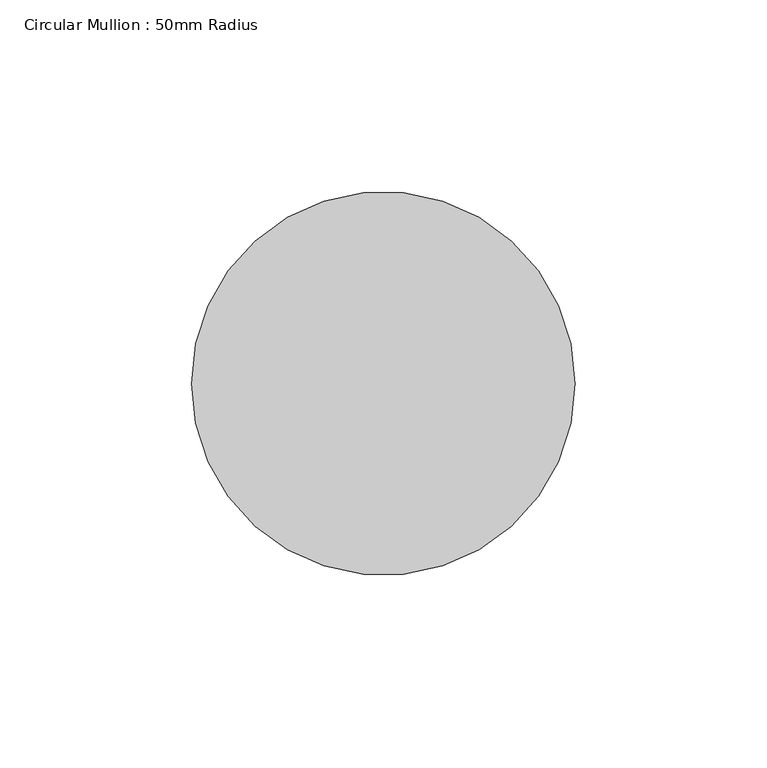
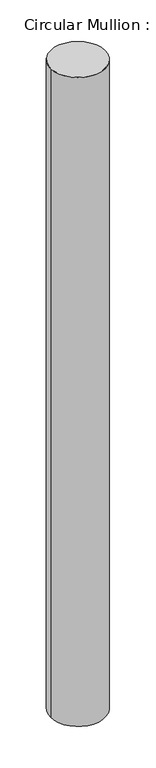
"""IFC4 building model written with IfcOpenShell, lengths in millimetres: member geometry, Circular Mullion : 50mm Radius."""

import ifcopenshell
import ifcopenshell.guid

model = None  # the IFC model being written
_history = None  # IfcOwnerHistory: only IFC2X3 demands one
_inside = {}  # id of a spatial element -> (the spatial element, [elements in it])
_under = {}  # id of a project, library or spatial element -> (it, [spatial elements below it])
_declared = {}  # id of a project -> (the project, [libraries it declares])
_typed = {}  # id of a type object -> (the type object, [elements of that type])
_made_of = {}  # id of a material, layer set ... -> (it, [elements and type objects made of it])


def new_model(schema):
    """Start an empty IFC model of exactly this schema.

    Asked for "IFC4X3", IfcOpenShell would pick the latest addendum, in which some entities
    have other attributes; the version numbers below select the first issue.
    IFC2X3 requires an IfcOwnerHistory on every rooted entity: one is made here for all.
    """
    global model, _history
    if schema == "IFC4X3":
        model = ifcopenshell.file(schema_version=(4, 3, 0, 0))
    else:
        model = ifcopenshell.file(schema=schema)
    _inside.clear()
    _under.clear()
    _declared.clear()
    _typed.clear()
    _made_of.clear()
    _history = None
    if model.schema == "IFC2X3":
        org = make("IfcOrganization", Name="unknown")
        user = make(
            "IfcPersonAndOrganization",
            ThePerson=make("IfcPerson", FamilyName="unknown"),
            TheOrganization=org,
        )
        app = make(
            "IfcApplication",
            ApplicationDeveloper=org,
            Version="unknown",
            ApplicationFullName="unknown",
            ApplicationIdentifier="unknown",
        )
        _history = make(
            "IfcOwnerHistory",
            OwningUser=user,
            OwningApplication=app,
            ChangeAction="ADDED",
            CreationDate=0,
        )
    return model


def make(cls, **values):
    """One entity of the class cls with the attributes given. An attribute that is None is left unset."""
    return model.create_entity(
        cls, **{name: value for name, value in values.items() if value is not None}
    )


def rooted(cls, **values):
    """An entity with a GlobalId (a new one), such as an element, a storey or a relation."""
    return make(cls, GlobalId=ifcopenshell.guid.new(), OwnerHistory=_history, **values)


def si_unit(unit_type, name, prefix=None):
    """IfcSIUnit, for example si_unit("LENGTHUNIT", "METRE", prefix="MILLI")."""
    return make("IfcSIUnit", UnitType=unit_type, Prefix=prefix, Name=name)


def assignment(units):
    """IfcUnitAssignment: the units of a project."""
    return None if units is None else make("IfcUnitAssignment", Units=units)


def point(xyz):
    """IfcCartesianPoint."""
    return None if xyz is None else make("IfcCartesianPoint", Coordinates=xyz)


def direction(xyz):
    """IfcDirection."""
    return None if xyz is None else make("IfcDirection", DirectionRatios=xyz)


def frame(location, z_axis=None, x_axis=None):
    """IfcAxis2Placement3D, a coordinate frame: its origin and axes. An axis left out is left unset."""
    return make(
        "IfcAxis2Placement3D",
        Location=point(location),
        Axis=direction(z_axis),
        RefDirection=direction(x_axis),
    )


def frame_2d(location, x_axis=None):
    """IfcAxis2Placement2D, a coordinate frame in the plane: its origin and x axis."""
    return make(
        "IfcAxis2Placement2D", Location=point(location), RefDirection=direction(x_axis)
    )


def origin():
    """The frame at (0, 0, 0) with its axes left unset."""
    return frame((0.0, 0.0, 0.0))


def origin_2d():
    """The frame at (0, 0) in the plane with its x axis left unset."""
    return frame_2d((0.0, 0.0))


def place(relative_to, where):
    """IfcLocalPlacement: puts the frame where relative to a parent placement (None: the world)."""
    return make(
        "IfcLocalPlacement", PlacementRelTo=relative_to, RelativePlacement=where
    )


def context(
    kind, dimensions, precision=None, world=None, true_north=None, identifier=None
):
    """IfcGeometricRepresentationContext, for example the 3D "Model" context."""
    return make(
        "IfcGeometricRepresentationContext",
        ContextIdentifier=identifier,
        ContextType=kind,
        CoordinateSpaceDimension=dimensions,
        Precision=precision,
        WorldCoordinateSystem=world,
        TrueNorth=true_north,
    )


def project(units=None, contexts=None):
    """IfcProject with its units and contexts."""
    return rooted(
        "IfcProject",
        Name="project",
        RepresentationContexts=contexts,
        UnitsInContext=assignment(units),
    )


def spatial(cls, under=None, at=None, **own):
    """A site, building, storey or space (cls), placed at a placement, below another one or the project."""
    s = rooted(cls, ObjectPlacement=at, **own)
    if under is not None:
        _under.setdefault(under.id(), (under, []))[1].append(s)
    return s


def circle_curve(where, radius):
    """IfcCircle in the frame where."""
    return make("IfcCircle", Position=where, Radius=radius)


def trimmed(basis, trim1, trim2, sense, master):
    """IfcTrimmedCurve: the piece of a basis curve between two trims."""
    return make(
        "IfcTrimmedCurve",
        BasisCurve=basis,
        Trim1=trim1,
        Trim2=trim2,
        SenseAgreement=sense,
        MasterRepresentation=master,
    )


def segment(curve, same_sense, transition):
    """IfcCompositeCurveSegment."""
    return make(
        "IfcCompositeCurveSegment",
        Transition=transition,
        SameSense=same_sense,
        ParentCurve=curve,
    )


def composite_curve(segments, self_intersect=None):
    """IfcCompositeCurve: segments joined end to end."""
    return make("IfcCompositeCurve", Segments=segments, SelfIntersect=self_intersect)


def outline(outer, holes=None, kind="AREA"):
    """IfcArbitraryClosedProfileDef: a profile drawn as a closed curve; with holes, ...WithVoids."""
    if holes is None:
        return make("IfcArbitraryClosedProfileDef", ProfileType=kind, OuterCurve=outer)
    return make(
        "IfcArbitraryProfileDefWithVoids",
        ProfileType=kind,
        OuterCurve=outer,
        InnerCurves=holes,
    )


def extrude(swept, where, along, depth):
    """IfcExtrudedAreaSolid: the profile swept, set in the frame where, extruded along a direction by depth."""
    return make(
        "IfcExtrudedAreaSolid",
        SweptArea=swept,
        Position=where,
        ExtrudedDirection=direction(along),
        Depth=depth,
    )


def shape(context_of_items, identifier, shape_type, items):
    """IfcShapeRepresentation: the items that make up one representation, for example the "Body"."""
    return make(
        "IfcShapeRepresentation",
        ContextOfItems=context_of_items,
        RepresentationIdentifier=identifier,
        RepresentationType=shape_type,
        Items=items,
    )


def source(mapping_origin, context_of_items, identifier, shape_type, items):
    """IfcRepresentationMap: a shape defined once, which mapped items show again and again."""
    return make(
        "IfcRepresentationMap",
        MappingOrigin=mapping_origin,
        MappedRepresentation=shape(context_of_items, identifier, shape_type, items),
    )


def transform(
    local_origin,
    x_axis=None,
    y_axis=None,
    z_axis=None,
    scale=None,
    scale2=None,
    scale3=None,
    uniform=True,
):
    """IfcCartesianTransformationOperator3D, or its non-uniform kind. x_axis, y_axis, z_axis: its Axis1, 2, 3."""
    if uniform:
        return make(
            "IfcCartesianTransformationOperator3D",
            Axis1=direction(x_axis),
            Axis2=direction(y_axis),
            LocalOrigin=point(local_origin),
            Scale=scale,
            Axis3=direction(z_axis),
        )
    return make(
        "IfcCartesianTransformationOperator3DnonUniform",
        Axis1=direction(x_axis),
        Axis2=direction(y_axis),
        LocalOrigin=point(local_origin),
        Scale=scale,
        Axis3=direction(z_axis),
        Scale2=scale2,
        Scale3=scale3,
    )


def mapped(mapping_source, mapping_target):
    """IfcMappedItem: shows the shape of a source again, moved by a transform."""
    return make(
        "IfcMappedItem", MappingSource=mapping_source, MappingTarget=mapping_target
    )


def made_of(thing, what):
    """Note that an element or type object is made of a material, layer set ...; save() writes the relation."""
    if what is not None:
        _made_of.setdefault(what.id(), (what, []))[1].append(thing)
    return thing


def element(
    cls,
    number,
    at=None,
    inside=None,
    cuts=None,
    type_object=None,
    material=None,
    context=None,
    identifier="Body",
    shape_type=None,
    held_by="IfcProductDefinitionShape",
    body=None,
    shapes=None,
    **own,
):
    """One element of the class cls, such as IfcWall. Its Tag is "e" and its number.

    at: its placement. inside: the storey or other place that contains it. cuts: it is an
    opening in that element (IfcRelVoidsElement). A single representation is given by context,
    identifier, shape_type and body (its items); several are given by shapes. held_by: the class
    of the entity that holds the representations. save() writes the other relations.
    """
    e = rooted(cls, Tag="e%d" % number, ObjectPlacement=at, **own)
    if body is not None:
        shapes = [shape(context, identifier, shape_type, body)]
    if shapes is not None:
        e.Representation = make(held_by, Representations=shapes)
    if inside is not None:
        _inside.setdefault(inside.id(), (inside, []))[1].append(e)
    if cuts is not None:
        rooted(
            "IfcRelVoidsElement", RelatingBuildingElement=cuts, RelatedOpeningElement=e
        )
    if type_object is not None:
        _typed.setdefault(type_object.id(), (type_object, []))[1].append(e)
    return made_of(e, material)


def aggregate(whole, parts):
    """IfcRelAggregates: a whole, such as a stair, and the parts it consists of."""
    return rooted("IfcRelAggregates", RelatingObject=whole, RelatedObjects=parts)


def save(model, path):
    """Write the relations noted so far, then the file.

    IfcRelAggregates (storeys below a building ...), IfcRelContainedInSpatialStructure (elements
    in a storey), IfcRelDefinesByType, IfcRelAssociatesMaterial and IfcRelDeclares: one each for
    every whole, place, type object, material and project.
    """
    for whole, parts in _under.values():
        aggregate(whole, parts)
    for where, things in _inside.values():
        rooted(
            "IfcRelContainedInSpatialStructure",
            RelatedElements=things,
            RelatingStructure=where,
        )
    for kind, things in _typed.values():
        rooted("IfcRelDefinesByType", RelatedObjects=things, RelatingType=kind)
    for what, things in _made_of.values():
        rooted("IfcRelAssociatesMaterial", RelatedObjects=things, RelatingMaterial=what)
    for by, libraries in _declared.values():
        rooted("IfcRelDeclares", RelatingContext=by, RelatedDefinitions=libraries)
    model.write(path)


def circular_mullion_50mm_radius_5b0c1a44(model_context):
    return source(origin(), model_context, "Body", "SweptSolid", [
        extrude(outline(composite_curve([segment(trimmed(circle_curve(origin_2d(), 50.0), [point((50.0, 0.0))], [point((-50.0, 0.0))], False, "CARTESIAN"), True, "CONTINUOUS"), segment(trimmed(circle_curve(origin_2d(), 50.0), [point((-50.0, 0.0))], [point((50.0, 0.0))], False, "CARTESIAN"), True, "CONTINUOUS")], self_intersect=False)), frame((0.0, 0.0, -1261.2140216), z_axis=(0.0, 0.0, 1.0), x_axis=(1.0, 0.0, 0.0)), (0.0, 0.0, 1.0), 1261.2140216),
    ])


if __name__ == "__main__":
    model = new_model("IFC4")
    model_context = context("Model", 3, world=origin())
    ifc_project = project(units=[si_unit("LENGTHUNIT", "METRE", prefix="MILLI")], contexts=[model_context])
    site = spatial("IfcSite", under=ifc_project)
    building = spatial("IfcBuilding", under=site)
    placement = place(None, origin())
    circular_mullion_50mm_radius_shape = circular_mullion_50mm_radius_5b0c1a44(model_context)
    element("IfcMember", 1, ObjectType="Circular Mullion : 50mm Radius", at=placement, inside=building, context=model_context, shape_type="MappedRepresentation", body=[
        mapped(circular_mullion_50mm_radius_shape, transform((0.0, 0.0, 0.0), x_axis=(1.0, 0.0, 0.0), y_axis=(0.0, 1.0, 0.0), z_axis=(0.0, 0.0, 1.0))),
    ])
    save(model, "model.ifc")

# Revit data of these elements
# Type "Circular Mullion : 50mm Radius"
#   built-in parameter 1007350 = 0.164042 (stored number, unit not read)
# Element 1 (IfcMember, "Circular Mullion : 50mm Radius")
#   Materials on its faces: "Aluminium"
# Materials
#   "Aluminium": class "Metal", colour RGB 247 247 247, transparency 0, Description = "Aluminium 6061", Cost = 0
